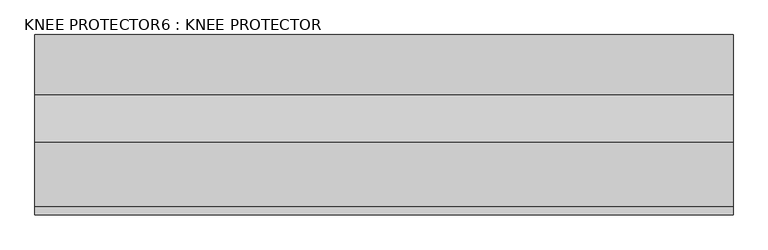
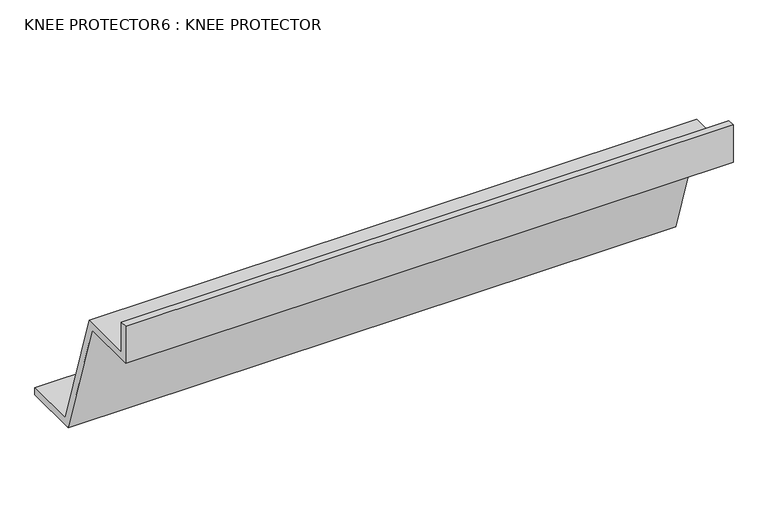
"""IFC4 building model written with IfcOpenShell, lengths in millimetres: furniture geometry, KNEE PROTECTOR6 : KNEE PROTECTOR."""

from ifc_helpers import new_model, si_unit, frame, origin, place, context, project, spatial, polyline, outline, extrude, source, transform, mapped, element, save


def knee_protector6_knee_protector_b4004326(model_context):
    return source(origin(), model_context, "Body", "SweptSolid", [
        extrude(outline(polyline([(-237028.2315414, 685.8), (-237028.2315414, 825.5), (-237002.8315414, 825.5), (-237002.8315414, 711.2), (-236803.9902606, 711.2), (-236655.4369755, 254.0), (-236469.4315414, 254.0), (-236469.4315414, 228.6), (-236673.8911557, 228.6), (-236822.4444408, 685.8), (-237028.2315414, 685.8)])), frame((-716725.3228174, 0.0, 0.0), z_axis=(1.0, 0.0, 0.0), x_axis=(0.0, 1.0, 0.0)), (0.0, 0.0, 1.0), 2162.175),
    ])


if __name__ == "__main__":
    model = new_model("IFC4")
    model_context = context("Model", 3, world=origin())
    ifc_project = project(units=[si_unit("LENGTHUNIT", "METRE", prefix="MILLI")], contexts=[model_context])
    site = spatial("IfcSite", under=ifc_project)
    building = spatial("IfcBuilding", under=site)
    placement = place(None, origin())
    knee_protector6_knee_protector_shape = knee_protector6_knee_protector_b4004326(model_context)
    element("IfcFurniture", 1, ObjectType="KNEE PROTECTOR6 : KNEE PROTECTOR", at=placement, inside=building, context=model_context, shape_type="MappedRepresentation", body=[
        mapped(knee_protector6_knee_protector_shape, transform((0.0, 0.0, 0.0), x_axis=(1.0, 0.0, 0.0), y_axis=(0.0, 1.0, 0.0), z_axis=(0.0, 0.0, 1.0))),
    ])
    save(model, "model.ifc")
